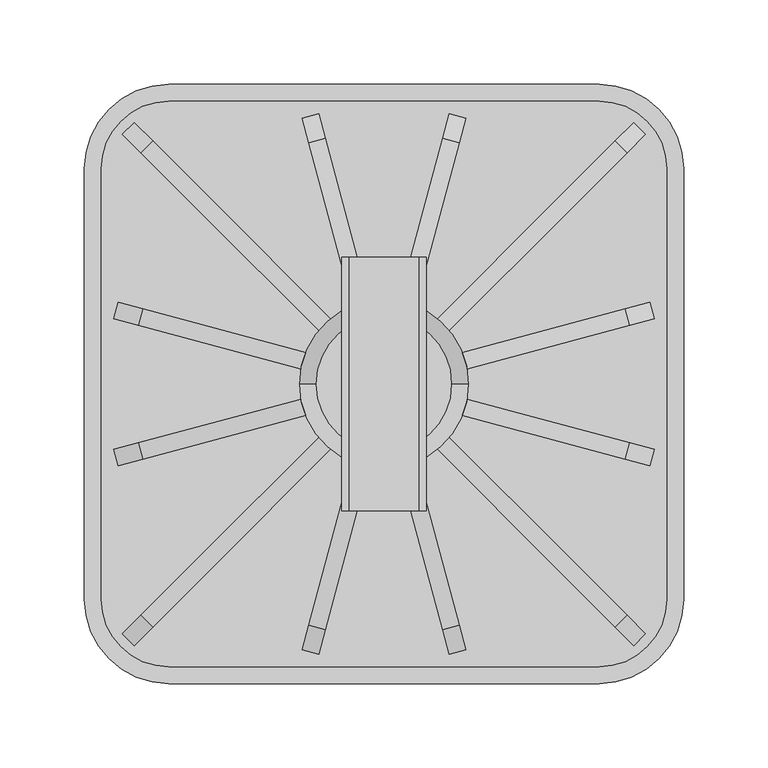
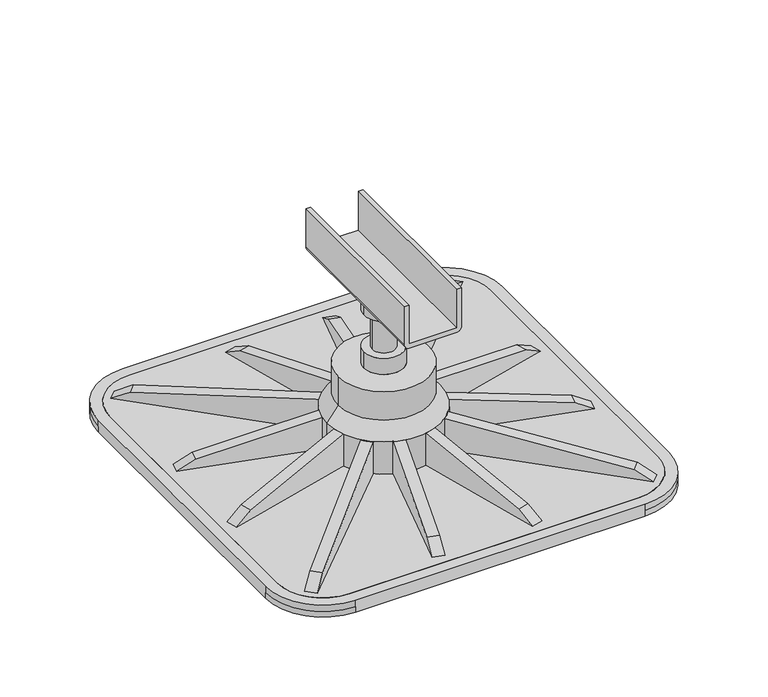
"""IFC4 building model written with IfcOpenShell, lengths in millimetres: proxy geometry, TN_Кровельная опора ТехноНИКОЛЬ : Кровельная опора ТехноНИКОЛЬ 355х355мм с горизонтальным кронштейном."""

from ifc_helpers import new_model, si_unit, point, frame, frame_2d, origin, origin_2d, place, context, project, spatial, polyline, circle_curve, trimmed, segment, composite_curve, outline, extrude, source, transform, mapped, element, save
from ifc_brep_helpers import plane_surface, cylinder_surface, revolved_surface, advanced_brep


def generic_models_53b3d343(model_context):
    return source(origin(), model_context, "Body", "SolidModel", [
        extrude(outline(polyline([(214.1306058, 0.0), (198.8913097, -8.6706701), (0.0, -35.5445162), (0.0, 0.0), (214.1306058, 0.0)])), frame((-3.5355339, -3.5355339, 11.0), z_axis=(0.7071067811865469, 0.7071067811865482, 0.0), x_axis=(0.7071067811865482, -0.7071067811865469, 0.0)), (0.0, 0.0, 1.0), 10.0),
        extrude(outline(polyline([(0.0, 0.0), (17.5333016, 1e-07), (203.6920691, -74.9991329), (186.1143887, -105.8931094), (0.0, 0.0)])), frame((154.9487373, 147.8776695, 11.0), z_axis=(-0.707106781186547, 0.7071067811865481, 0.0), x_axis=(-0.6145910150795418, -0.6145910150795407, 0.49452580151797754)), (0.0, 0.0, 1.0), 10.0),
        extrude(outline(polyline([(-214.1306058, 0.0), (0.0, 0.0), (0.0, -35.5445162), (-198.8913097, -8.6706701), (-214.1306058, 0.0)])), frame((-3.5355339, -3.5355339, 11.0), z_axis=(0.7071067811865469, 0.7071067811865482, 0.0), x_axis=(0.7071067811865482, -0.7071067811865469, 0.0)), (0.0, 0.0, 1.0), 10.0),
        extrude(outline(polyline([(0.0, 0.0), (-142.9576707, -80.9713708), (-162.6162897, -46.2634197), (-17.1780129, 0.0), (0.0, 0.0)])), frame((-38.6654497, -159.9920884, 11.0), z_axis=(-0.9659258262890678, 0.25881904510252296, 0.0), x_axis=(-0.22520396734385073, -0.8404726481933256, -0.4928376007687403)), (0.0, 0.0, 1.0), 10.0),
        extrude(outline(polyline([(164.4678969, 0.0), (149.5209418, -8.4659707), (0.1716447, -39.8886346), (0.1716447, 0.0), (164.4678969, 0.0)])), frame((-3.9019744, -1.1282992, 11.0), z_axis=(0.9659258262890678, 0.25881904510252296, 0.0), x_axis=(0.25881904510252296, -0.9659258262890678, 0.0)), (0.0, 0.0, 1.0), 10.0),
        extrude(outline(polyline([(0.0, 0.0), (17.1780129, 0.0), (162.6162896, -46.2634196), (142.9576706, -80.9713707), (0.0, 0.0)])), frame((157.4038979, -48.3247079, 11.0), z_axis=(0.2588190451025272, 0.9659258262890665, 0.0), x_axis=(-0.8404726481933232, 0.22520396734385406, 0.4928376007687429)), (0.0, 0.0, 1.0), 10.0),
        extrude(outline(polyline([(164.4678969, 0.0), (149.5209418, -8.4659707), (0.1716447, -39.8886346), (0.1716447, 0.0), (164.4678969, 0.0)])), frame((1.1282992, -3.9019744, 11.0), z_axis=(-0.25881904510252723, 0.9659258262890665, 0.0), x_axis=(0.9659258262890665, 0.25881904510252723, 0.0)), (0.0, 0.0, 1.0), 10.0),
        extrude(outline(polyline([(0.0, 0.0), (17.1780129, 0.0), (162.6162896, -46.2634196), (142.9576706, -80.9713707), (0.0, 0.0)])), frame((48.3247079, 157.4038979, 11.0), z_axis=(-0.9659258262890661, 0.2588190451025289, 0.0), x_axis=(-0.22520396734385595, -0.8404726481933242, 0.4928376007687402)), (0.0, 0.0, 1.0), 10.0),
        extrude(outline(polyline([(-164.4678969, 0.0), (-0.1716447, 0.0), (-0.1716447, -39.8886346), (-149.5209418, -8.4659707), (-164.4678969, 0.0)])), frame((-5.7572839, -1.4598913, 11.0), z_axis=(0.9659258262890661, 0.25881904510252896, 0.0), x_axis=(0.25881904510252896, -0.9659258262890661, 0.0)), (0.0, 0.0, 1.0), 10.0),
        extrude(outline(polyline([(0.0, 0.0), (-142.9576707, -80.9713708), (-162.6162897, -46.2634197), (-17.1780129, 0.0), (0.0, 0.0)])), frame((-159.9920884, 38.6654497, 11.0), z_axis=(0.25881904510253323, 0.9659258262890649, 0.0), x_axis=(-0.8404726481933251, 0.2252039673438602, -0.4928376007687367)), (0.0, 0.0, 1.0), 10.0),
        extrude(outline(composite_curve([segment(trimmed(circle_curve(origin_2d(), 17.25), [point((-17.25, 0.0))], [point((17.25, 0.0))], False, "CARTESIAN"), True, "CONTINUOUS"), segment(trimmed(circle_curve(origin_2d(), 17.25), [point((17.25, 0.0))], [point((-17.25, 0.0))], False, "CARTESIAN"), True, "CONTINUOUS")], self_intersect=False)), frame((0.0, 0.0, 130.0), z_axis=(0.0, 0.0, 1.0), x_axis=(1.0, 0.0, 0.0)), (0.0, 0.0, 1.0), 16.0),
        extrude(outline(composite_curve([segment(trimmed(circle_curve(frame_2d((150.0, -21.0)), 4.0), [point((150.0, -25.0))], [point((146.0, -21.0))], False, "CARTESIAN"), True, "CONTINUOUS"), segment(polyline([(146.0, -21.0), (146.0, 21.0)]), True, "CONTINUOUS"), segment(trimmed(circle_curve(frame_2d((150.0, 21.0)), 4.0), [point((146.0, 21.0))], [point((150.0, 25.0))], False, "CARTESIAN"), True, "CONTINUOUS"), segment(polyline([(150.0, 25.0), (186.0, 25.0), (186.0, 21.0), (150.0, 21.0), (150.0, -21.0), (186.0, -21.0), (186.0, -25.0), (150.0, -25.0)]), True, "CONTINUOUS")], self_intersect=False)), frame((0.0, -75.0, 0.0), z_axis=(0.0, 1.0, 0.0), x_axis=(0.0, 0.0, 1.0)), (0.0, 0.0, 1.0), 150.0),
        advanced_brep(
        [(-40.0, 0.0, 80.6), (40.0, 0.0, 80.6), (17.25, 0.0, 80.6), (-17.25, 0.0, 80.6), (-40.0, 0.0, 54.2), (40.0, 0.0, 54.2), (-10.0, 0.0, 146.0), (10.0, 0.0, 146.0), (-10.0, 0.0, 95.6), (10.0, 0.0, 95.6), (-17.25, 0.0, 95.6), (17.25, 0.0, 95.6)],
        [
            (0, 1, circle_curve(frame((0.0, 0.0, 80.6), z_axis=(0.0, 0.0, 1.0), x_axis=(1.0, 0.0, 0.0)), 40.0)),
            (1, 0, circle_curve(frame((0.0, 0.0, 80.6), z_axis=(0.0, 0.0, 1.0), x_axis=(1.0, 0.0, 0.0)), 40.0)),
            (2, 3, circle_curve(frame((0.0, 0.0, 80.6), z_axis=(0.0, 0.0, -1.0), x_axis=(1.0, 0.0, 0.0)), 17.25)),
            (3, 2, circle_curve(frame((0.0, 0.0, 80.6), z_axis=(0.0, 0.0, -1.0), x_axis=(1.0, 0.0, 0.0)), 17.25)),
            (4, 5, circle_curve(frame((0.0, 0.0, 54.2), z_axis=(0.0, 0.0, -1.0), x_axis=(1.0, 0.0, 0.0)), 40.0)),
            (5, 4, circle_curve(frame((0.0, 0.0, 54.2), z_axis=(0.0, 0.0, -1.0), x_axis=(1.0, 0.0, 0.0)), 40.0)),
            (0, 4),
            (5, 1),
            (6, 7, circle_curve(frame((0.0, 0.0, 146.0), z_axis=(0.0, 0.0, 1.0), x_axis=(1.0, 0.0, 0.0)), 10.0)),
            (7, 6, circle_curve(frame((0.0, 0.0, 146.0), z_axis=(0.0, 0.0, 1.0), x_axis=(1.0, 0.0, 0.0)), 10.0)),
            (6, 8),
            (8, 9, circle_curve(frame((0.0, 0.0, 95.6), z_axis=(0.0, 0.0, 1.0), x_axis=(1.0, 0.0, 0.0)), 10.0)),
            (9, 7),
            (9, 8, circle_curve(frame((0.0, 0.0, 95.6), z_axis=(0.0, 0.0, 1.0), x_axis=(1.0, 0.0, 0.0)), 10.0)),
            (10, 11, circle_curve(frame((0.0, 0.0, 95.6), z_axis=(0.0, 0.0, 1.0), x_axis=(1.0, 0.0, 0.0)), 17.25)),
            (11, 10, circle_curve(frame((0.0, 0.0, 95.6), z_axis=(0.0, 0.0, 1.0), x_axis=(1.0, 0.0, 0.0)), 17.25)),
            (10, 3),
            (2, 11),
        ],
        [
            plane_surface(frame((40.0, 0.0, 80.6), z_axis=(0.0, 0.0, 1.0), x_axis=(0.0, 1.0, 0.0))),
            plane_surface(frame((40.0, 0.0, 54.2), z_axis=(0.0, 0.0, -1.0), x_axis=(0.0, -1.0, 0.0))),
            cylinder_surface(frame((0.0, 0.0, 54.2), z_axis=(0.0, 0.0, 1.0), x_axis=(1.0, 0.0, 0.0)), 40.0),
            plane_surface(frame((10.0, 0.0, 146.0), z_axis=(0.0, 0.0, 1.0), x_axis=(0.0, 1.0, 0.0))),
            cylinder_surface(frame((0.0, 0.0, 80.6), z_axis=(0.0, 0.0, 1.0), x_axis=(1.0, 0.0, 0.0)), 10.0),
            plane_surface(frame((17.25, 0.0, 95.6), z_axis=(0.0, 0.0, 1.0), x_axis=(0.0, 1.0, 0.0))),
            cylinder_surface(frame((0.0, 0.0, 80.6), z_axis=(0.0, 0.0, 1.0), x_axis=(1.0, 0.0, 0.0)), 17.25),
        ],
        [
            (0, [[1, 2], [3, 4]]),
            (1, [[5, 6]]),
            (2, [[-1, 7, -6, 8]]),
            (2, [[-2, -8, -5, -7]]),
            (3, [[9, 10]]),
            (4, [[-9, 11, 12, 13]]),
            (4, [[-10, -13, 14, -11]]),
            (5, [[15, 16], [-12, -14]]),
            (6, [[-15, 17, -3, 18]]),
            (6, [[-16, -18, -4, -17]]),
        ],
    ),
        extrude(outline(polyline([(-164.4678969, 0.0), (-0.1716447, 0.0), (-0.1716447, -39.8886346), (-149.5209418, -8.4659707), (-164.4678969, 0.0)])), frame((1.4598913, -5.7572839, 11.0), z_axis=(-0.25881904510253323, 0.965925826289065, 0.0), x_axis=(0.965925826289065, 0.25881904510253323, 0.0)), (0.0, 0.0, 1.0), 10.0),
        extrude(outline(polyline([(0.0, 0.0), (-186.1143887, -105.8931094), (-203.6920691, -74.9991329), (-17.5333016, 1e-07), (0.0, 0.0)])), frame((-147.8776695, -154.9487373, 11.0), z_axis=(-0.7071067811865469, 0.7071067811865482, 0.0), x_axis=(-0.6145910150795192, -0.6145910150795181, -0.4945258015180338)), (0.0, 0.0, 1.0), 10.0),
        advanced_brep(
        [(-40.0, 0.0, 54.2), (40.0, 0.0, 54.2), (-50.0, 0.0, 41.0), (50.0, 0.0, 41.0)],
        [
            (0, 1, circle_curve(frame((0.0, 0.0, 54.2), z_axis=(0.0, 0.0, 1.0), x_axis=(-1.0, 0.0, 0.0)), 40.0)),
            (1, 0, circle_curve(frame((0.0, 0.0, 54.2), z_axis=(0.0, 0.0, 1.0), x_axis=(1.0, 0.0, 0.0)), 40.0)),
            (2, 3, circle_curve(frame((0.0, 0.0, 41.0), z_axis=(0.0, 0.0, -1.0), x_axis=(1.0, 0.0, 0.0)), 50.0)),
            (3, 2, circle_curve(frame((0.0, 0.0, 41.0), z_axis=(0.0, 0.0, -1.0), x_axis=(-1.0, 0.0, 0.0)), 50.0)),
            (3, 1),
            (0, 2),
        ],
        [
            plane_surface(frame((0.0, 0.0, 54.2), z_axis=(0.0, 0.0, 1.0), x_axis=(0.0, -1.0, 0.0))),
            plane_surface(frame((0.0, 0.0, 41.0), z_axis=(0.0, 0.0, -1.0), x_axis=(0.0, -1.0, 0.0))),
            revolved_surface(polyline([(-40.0, 0.0, 54.2), (-50.0, 0.0, 41.0)]), (0.0, 0.0, 107.0), (0.0, 0.0, -1.0)),
            revolved_surface(polyline([(40.0, 0.0, 54.2), (50.0, 0.0, 41.0)]), (0.0, 0.0, 107.0), (0.0, 0.0, -1.0)),
        ],
        [
            (0, [[1, 2]]),
            (1, [[3, 4]]),
            (2, [[-4, 5, -1, 6]]),
            (3, [[-3, -6, -2, -5]]),
        ],
    ),
        extrude(outline(composite_curve([segment(trimmed(circle_curve(origin_2d(), 50.0), [point((-50.0, 0.0))], [point((50.0, 0.0))], False, "CARTESIAN"), True, "CONTINUOUS"), segment(trimmed(circle_curve(origin_2d(), 50.0), [point((50.0, 0.0))], [point((-50.0, 0.0))], False, "CARTESIAN"), True, "CONTINUOUS")], self_intersect=False)), frame((0.0, 0.0, 11.0), z_axis=(0.0, 0.0, 1.0), x_axis=(1.0, 0.0, 0.0)), (0.0, 0.0, 1.0), 30.0),
        extrude(outline(composite_curve([segment(trimmed(circle_curve(frame_2d((127.5, 127.5)), 40.0), [point((127.5, 167.5))], [point((167.5, 127.5))], False, "CARTESIAN"), True, "CONTINUOUS"), segment(polyline([(167.5, 127.5), (167.5, -127.5)]), True, "CONTINUOUS"), segment(trimmed(circle_curve(frame_2d((127.5, -127.5)), 40.0), [point((167.5, -127.5))], [point((127.5, -167.5))], False, "CARTESIAN"), True, "CONTINUOUS"), segment(polyline([(127.5, -167.5), (-127.5, -167.5)]), True, "CONTINUOUS"), segment(trimmed(circle_curve(frame_2d((-127.5, -127.5)), 40.0), [point((-127.5, -167.5))], [point((-167.5, -127.5))], False, "CARTESIAN"), True, "CONTINUOUS"), segment(polyline([(-167.5, -127.5), (-167.5, 127.5)]), True, "CONTINUOUS"), segment(trimmed(circle_curve(frame_2d((-127.5, 127.5)), 40.0), [point((-167.5, 127.5))], [point((-127.5, 167.5))], False, "CARTESIAN"), True, "CONTINUOUS"), segment(polyline([(-127.5, 167.5), (127.5, 167.5)]), True, "CONTINUOUS")], self_intersect=False)), frame((0.0, 0.0, 5.0), z_axis=(0.0, 0.0, 1.0), x_axis=(1.0, 0.0, 0.0)), (0.0, 0.0, 1.0), 6.0),
        advanced_brep(
        [(-127.5, 167.5, 5.0), (-167.5, 127.5, 5.0), (-167.5, -127.5, 5.0), (-127.5, -167.5, 5.0), (127.5, -167.5, 5.0), (167.5, -127.5, 5.0), (167.5, 127.5, 5.0), (127.5, 167.5, 5.0), (-177.5, -127.5, 0.0), (-177.5, 127.5, 0.0), (-127.5, 177.5, 0.0), (127.5, 177.5, 0.0), (177.5, 127.5, 0.0), (177.5, -127.5, 0.0), (127.5, -177.5, 0.0), (-127.5, -177.5, 0.0), (-127.5, -177.5, 5.0), (-177.5, -127.5, 5.0), (127.5, -177.5, 5.0), (127.5, -177.5, 11.0), (-127.5, -177.5, 11.0), (177.5, -127.5, 5.0), (177.5, 127.5, 5.0), (177.5, 127.5, 11.0), (177.5, -127.5, 11.0), (127.5, 177.5, 5.0), (-127.5, 177.5, 5.0), (-127.5, 177.5, 11.0), (127.5, 177.5, 11.0), (-177.5, 127.5, 5.0), (-177.5, -127.5, 11.0), (-177.5, 127.5, 11.0), (-167.5, 127.5, 11.0), (-127.5, 167.5, 11.0), (127.5, 167.5, 11.0), (167.5, 127.5, 11.0), (167.5, -127.5, 11.0), (127.5, -167.5, 11.0), (-127.5, -167.5, 11.0), (-167.5, -127.5, 11.0)],
        [
            (0, 1, circle_curve(frame((-127.5, 127.5, 5.0), z_axis=(0.0, 0.0, 1.0), x_axis=(1.0, 0.0, 0.0)), 40.0)),
            (1, 2),
            (2, 3, circle_curve(frame((-127.5, -127.5, 5.0), z_axis=(0.0, 0.0, 1.0), x_axis=(1.0, 0.0, 0.0)), 40.0)),
            (3, 4),
            (4, 5, circle_curve(frame((127.5, -127.5, 5.0), z_axis=(0.0, 0.0, 1.0), x_axis=(1.0, 0.0, 0.0)), 40.0)),
            (5, 6),
            (6, 7, circle_curve(frame((127.5, 127.5, 5.0), z_axis=(0.0, 0.0, 1.0), x_axis=(1.0, 0.0, 0.0)), 40.0)),
            (7, 0),
            (8, 9),
            (9, 10, circle_curve(frame((-127.5, 127.5, 0.0), z_axis=(0.0, 0.0, -1.0), x_axis=(1.0, 0.0, 0.0)), 50.0)),
            (10, 11),
            (11, 12, circle_curve(frame((127.5, 127.5, 0.0), z_axis=(0.0, 0.0, -1.0), x_axis=(1.0, 0.0, 0.0)), 50.0)),
            (12, 13),
            (13, 14, circle_curve(frame((127.5, -127.5, 0.0), z_axis=(0.0, 0.0, -1.0), x_axis=(1.0, 0.0, 0.0)), 50.0)),
            (14, 15),
            (15, 8, circle_curve(frame((-127.5, -127.5, 0.0), z_axis=(0.0, 0.0, -1.0), x_axis=(1.0, 0.0, 0.0)), 50.0)),
            (15, 16),
            (16, 17, circle_curve(frame((-127.5, -127.5, 5.0), z_axis=(0.0, 0.0, -1.0), x_axis=(1.0, 0.0, 0.0)), 50.0)),
            (17, 8),
            (14, 18),
            (18, 19),
            (19, 20),
            (20, 16),
            (13, 21),
            (21, 18, circle_curve(frame((127.5, -127.5, 5.0), z_axis=(0.0, 0.0, -1.0), x_axis=(1.0, 0.0, 0.0)), 50.0)),
            (12, 22),
            (22, 23),
            (23, 24),
            (24, 21),
            (11, 25),
            (25, 22, circle_curve(frame((127.5, 127.5, 5.0), z_axis=(0.0, 0.0, -1.0), x_axis=(1.0, 0.0, 0.0)), 50.0)),
            (10, 26),
            (26, 27),
            (27, 28),
            (28, 25),
            (9, 29),
            (29, 26, circle_curve(frame((-127.5, 127.5, 5.0), z_axis=(0.0, 0.0, -1.0), x_axis=(1.0, 0.0, 0.0)), 50.0)),
            (17, 30),
            (30, 31),
            (31, 29),
            (27, 31, circle_curve(frame((-127.5, 127.5, 11.0), z_axis=(0.0, 0.0, 1.0), x_axis=(1.0, 0.0, 0.0)), 50.0)),
            (30, 20, circle_curve(frame((-127.5, -127.5, 11.0), z_axis=(0.0, 0.0, 1.0), x_axis=(1.0, 0.0, 0.0)), 50.0)),
            (19, 24, circle_curve(frame((127.5, -127.5, 11.0), z_axis=(0.0, 0.0, 1.0), x_axis=(1.0, 0.0, 0.0)), 50.0)),
            (23, 28, circle_curve(frame((127.5, 127.5, 11.0), z_axis=(0.0, 0.0, 1.0), x_axis=(1.0, 0.0, 0.0)), 50.0)),
            (32, 33, circle_curve(frame((-127.5, 127.5, 11.0), z_axis=(0.0, 0.0, -1.0), x_axis=(1.0, 0.0, 0.0)), 40.0)),
            (33, 34),
            (34, 35, circle_curve(frame((127.5, 127.5, 11.0), z_axis=(0.0, 0.0, -1.0), x_axis=(1.0, 0.0, 0.0)), 40.0)),
            (35, 36),
            (36, 37, circle_curve(frame((127.5, -127.5, 11.0), z_axis=(0.0, 0.0, -1.0), x_axis=(1.0, 0.0, 0.0)), 40.0)),
            (37, 38),
            (38, 39, circle_curve(frame((-127.5, -127.5, 11.0), z_axis=(0.0, 0.0, -1.0), x_axis=(1.0, 0.0, 0.0)), 40.0)),
            (39, 32),
            (32, 1),
            (0, 33),
            (7, 34),
            (6, 35),
            (5, 36),
            (4, 37),
            (3, 38),
            (2, 39),
        ],
        [
            plane_surface(frame((-77.5, -127.5, 5.0), z_axis=(0.0, 0.0, 1.0), x_axis=(0.0, 1.0, 0.0))),
            plane_surface(frame((-77.5, -127.5, 0.0), z_axis=(0.0, 0.0, -1.0), x_axis=(0.0, -1.0, 0.0))),
            cylinder_surface(frame((-127.5, -127.5, 0.0), z_axis=(0.0, 0.0, 1.0), x_axis=(1.0, 0.0, 0.0)), 50.0),
            plane_surface(frame((-127.5, -177.5, 5.0), z_axis=(0.0, -1.0, 0.0), x_axis=(0.0, 0.0, -1.0))),
            cylinder_surface(frame((127.5, -127.5, 0.0), z_axis=(0.0, 0.0, 1.0), x_axis=(1.0, 0.0, 0.0)), 50.0),
            plane_surface(frame((177.5, -127.5, 5.0), z_axis=(1.0, 0.0, 0.0), x_axis=(0.0, 0.0, -1.0))),
            cylinder_surface(frame((127.5, 127.5, 0.0), z_axis=(0.0, 0.0, 1.0), x_axis=(1.0, 0.0, 0.0)), 50.0),
            plane_surface(frame((127.5, 177.5, 5.0), z_axis=(0.0, 1.0, 0.0), x_axis=(0.0, 0.0, -1.0))),
            cylinder_surface(frame((-127.5, 127.5, 0.0), z_axis=(0.0, 0.0, 1.0), x_axis=(1.0, 0.0, 0.0)), 50.0),
            plane_surface(frame((-177.5, 127.5, 5.0), z_axis=(-1.0, 0.0, 0.0), x_axis=(0.0, 0.0, -1.0))),
            plane_surface(frame((-77.5, 127.5, 11.0), z_axis=(0.0, 0.0, 1.0), x_axis=(0.0, 1.0, 0.0))),
            cylinder_surface(frame((-127.5, 127.5, 5.0), z_axis=(0.0, 0.0, 1.0), x_axis=(1.0, 0.0, 0.0)), 50.0),
            cylinder_surface(frame((-127.5, -127.5, 5.0), z_axis=(0.0, 0.0, 1.0), x_axis=(1.0, 0.0, 0.0)), 50.0),
            cylinder_surface(frame((127.5, -127.5, 5.0), z_axis=(0.0, 0.0, 1.0), x_axis=(1.0, 0.0, 0.0)), 50.0),
            cylinder_surface(frame((127.5, 127.5, 5.0), z_axis=(0.0, 0.0, 1.0), x_axis=(1.0, 0.0, 0.0)), 50.0),
            revolved_surface(polyline([(-87.5, 127.5, 5.0), (-87.5, 127.5, 11.0)]), (-127.5, 127.5, 0.0), (0.0, 0.0, -1.0)),
            plane_surface(frame((-127.5, 167.5, 11.0), z_axis=(0.0, -1.0, 0.0), x_axis=(0.0, 0.0, -1.0))),
            revolved_surface(polyline([(167.5, 127.5, 5.0), (167.5, 127.5, 11.0)]), (127.5, 127.5, 0.0), (0.0, 0.0, -1.0)),
            plane_surface(frame((167.5, 127.5, 11.0), z_axis=(-1.0, 0.0, 0.0), x_axis=(0.0, 0.0, -1.0))),
            revolved_surface(polyline([(167.5, -127.5, 5.0), (167.5, -127.5, 11.0)]), (127.5, -127.5, 0.0), (0.0, 0.0, -1.0)),
            plane_surface(frame((127.5, -167.5, 11.0), z_axis=(0.0, 1.0, 0.0), x_axis=(0.0, 0.0, -1.0))),
            revolved_surface(polyline([(-87.5, -127.5, 5.0), (-87.5, -127.5, 11.0)]), (-127.5, -127.5, 0.0), (0.0, 0.0, -1.0)),
            plane_surface(frame((-167.5, -127.5, 11.0), z_axis=(1.0, 0.0, 0.0), x_axis=(0.0, 0.0, -1.0))),
        ],
        [
            (0, [[1, 2, 3, 4, 5, 6, 7, 8]]),
            (1, [[9, 10, 11, 12, 13, 14, 15, 16]]),
            (2, [[-16, 17, 18, 19]]),
            (3, [[-15, 20, 21, 22, 23, -17]]),
            (4, [[-14, 24, 25, -20]]),
            (5, [[-13, 26, 27, 28, 29, -24]]),
            (6, [[-12, 30, 31, -26]]),
            (7, [[-11, 32, 33, 34, 35, -30]]),
            (8, [[-10, 36, 37, -32]]),
            (9, [[-9, -19, 38, 39, 40, -36]]),
            (10, [[41, -39, 42, -22, 43, -28, 44, -34], [45, 46, 47, 48, 49, 50, 51, 52]]),
            (11, [[-41, -33, -37, -40]]),
            (12, [[-42, -38, -18, -23]]),
            (13, [[-43, -21, -25, -29]]),
            (14, [[-44, -27, -31, -35]]),
            (15, [[-45, 53, -1, 54]]),
            (16, [[-46, -54, -8, 55]]),
            (17, [[-47, -55, -7, 56]]),
            (18, [[-48, -56, -6, 57]]),
            (19, [[-49, -57, -5, 58]]),
            (20, [[-50, -58, -4, 59]]),
            (21, [[-51, -59, -3, 60]]),
            (22, [[-52, -60, -2, -53]]),
        ],
    ),
    ])


if __name__ == "__main__":
    model = new_model("IFC4")
    model_context = context("Model", 3, world=origin())
    ifc_project = project(units=[si_unit("LENGTHUNIT", "METRE", prefix="MILLI")], contexts=[model_context])
    site = spatial("IfcSite", under=ifc_project)
    building = spatial("IfcBuilding", under=site)
    placement = place(None, origin())
    generic_models_shape = generic_models_53b3d343(model_context)
    element("IfcBuildingElementProxy", 1, Name="TN_Кровельная опора ТехноНИКОЛЬ : Кровельная опора ТехноНИКОЛЬ 355х355мм с горизонтальным кронштейном", ObjectType="TN_Кровельная опора ТехноНИКОЛЬ : Кровельная опора ТехноНИКОЛЬ 355х355мм с горизонтальным кронштейном", at=placement, inside=building, context=model_context, shape_type="MappedRepresentation", body=[
        mapped(generic_models_shape, transform((0.0, 0.0, 0.0), x_axis=(1.0, 0.0, 0.0), y_axis=(0.0, 1.0, 0.0), z_axis=(0.0, 0.0, 1.0))),
    ])
    save(model, "model.ifc")

# Revit data of these elements
# Type "TN_Кровельная опора ТехноНИКОЛЬ : Кровельная опора ТехноНИКОЛЬ 355х355мм с горизонтальным кронштейном"
#   Description = "Кровельные опоры ТехноНИКОЛЬ, служат в качестве решение для размещения инженерных коммуникаций и промышленного оборудования на крыше здания, чиллеров, кондиционеров, воздуховодов, трубопроводов. Отличительной особенностью является регулировка кронштейна опоры, для необходимости компенсации уклона кровли."
#   Manufacturer = "ТехноНИКОЛЬ"
#   ADSK_Обозначение = "ТехноНИКОЛЬ"
#   ADSK_Наименование = "Кровельная опора ТехноНИКОЛЬ 355х355мм с горизонтальным кронштейном"
#   ADSK_Масса_Текст = ""
#   ADSK_Марка = "355х355"
#   ADSK_Код изделия = "43001"
#   ADSK_Завод-изготовитель = "ТехноНИКОЛЬ"
#   ADSK_Единица измерения = "шт."
#   ADSK_Группирование = "Комплектующие к опорам"
#   ADSK_URL страницы изделия = ""
#   ADSK_URL документации изделия = ""
#   ADSK_Размер_Ширина = 355 mm
#   ADSK_Масса = 0
#   ADSK_Количество = 1
#   Видимость_Кронштейн горизонтальный = yes
#   Видимость_Кронштейн вертикальный = no
#   ADSK_Материал = TN_Пластик_Красный
#   Default Elevation = 0
#   URL = ""
# Element 1 (IfcBuildingElementProxy, "TN_Кровельная опора ТехноНИКОЛЬ : Кровельная опора ТехноНИКОЛЬ 355х355мм с горизонтальным кронштейном")
#   Materials on its faces: "TN_Пластик_Красный", "TN_СтальГальванизированная_Серый", "TN_Пластик_ТемноСерый"
# Materials
#   "TN_Пластик_Красный": class "Типовые", colour RGB 200 10 50, transparency 0, Cost = 0
#   "TN_СтальГальванизированная_Серый": class "Типовые", colour RGB 206 210 213, transparency 0, Cost = 0
#   "TN_Пластик_ТемноСерый": class "Типовые", colour RGB 50 50 50, transparency 0, Cost = 0
